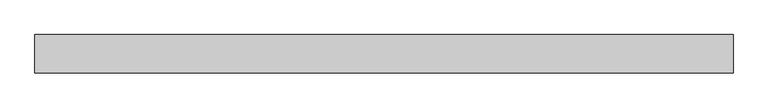
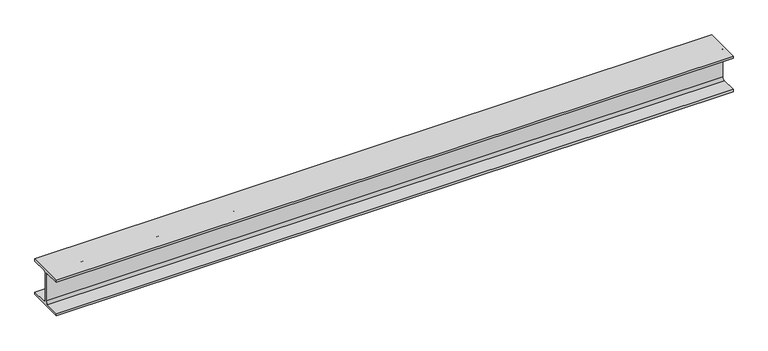
"""IFC4 building model written with IfcOpenShell, lengths in millimetres: beam geometry, 0912_Steel Framing_H-KSD3502 : H_SB_ASB_H-200x200x8x12."""

from ifc_helpers import new_model, si_unit, point, frame, frame_2d, origin, place, context, project, spatial, polyline, circle_curve, trimmed, segment, composite_curve, outline, extrude, source, transform, mapped, element, save


def beam_58b5673e(model_context):
    return source(origin(), model_context, "Body", "SweptSolid", [
        extrude(outline(composite_curve([segment(polyline([(100.0, -88.0), (100.0, -100.0), (-100.0, -100.0), (-100.0, -88.0), (-17.0, -88.0)]), True, "CONTINUOUS"), segment(trimmed(circle_curve(frame_2d((-17.0, -75.0)), 13.0), [point((-17.0, -88.0))], [point((-4.0, -75.0))], True, "CARTESIAN"), True, "CONTINUOUS"), segment(polyline([(-4.0, -75.0), (-4.0, 75.0)]), True, "CONTINUOUS"), segment(trimmed(circle_curve(frame_2d((-17.0, 75.0)), 13.0), [point((-4.0, 75.0))], [point((-17.0, 88.0))], True, "CARTESIAN"), True, "CONTINUOUS"), segment(polyline([(-17.0, 88.0), (-100.0, 88.0), (-100.0, 100.0), (100.0, 100.0), (100.0, 88.0), (17.0, 88.0)]), True, "CONTINUOUS"), segment(trimmed(circle_curve(frame_2d((17.0, 75.0)), 13.0), [point((17.0, 88.0))], [point((4.0, 75.0))], True, "CARTESIAN"), True, "CONTINUOUS"), segment(polyline([(4.0, 75.0), (4.0, -75.0)]), True, "CONTINUOUS"), segment(trimmed(circle_curve(frame_2d((17.0, -75.0)), 13.0), [point((4.0, -75.0))], [point((17.0, -88.0))], True, "CARTESIAN"), True, "CONTINUOUS"), segment(polyline([(17.0, -88.0), (100.0, -88.0)]), True, "CONTINUOUS")], self_intersect=False)), frame((-1850.8543264, 0.0, 0.0), z_axis=(1.0, 0.0, 0.0), x_axis=(0.0, 1.0, 0.0)), (0.0, 0.0, 1.0), 3630.9979746),
    ])


if __name__ == "__main__":
    model = new_model("IFC4")
    model_context = context("Model", 3, world=origin())
    ifc_project = project(units=[si_unit("LENGTHUNIT", "METRE", prefix="MILLI")], contexts=[model_context])
    site = spatial("IfcSite", under=ifc_project)
    building = spatial("IfcBuilding", under=site)
    placement = place(None, origin())
    beam_shape = beam_58b5673e(model_context)
    element("IfcBeam", 1, ObjectType="0912_Steel Framing_H-KSD3502 : H_SB_ASB_H-200x200x8x12", at=placement, inside=building, context=model_context, shape_type="MappedRepresentation", body=[
        mapped(beam_shape, transform((0.0, 0.0, 0.0), x_axis=(1.0, 0.0, 0.0), y_axis=(0.0, 1.0, 0.0), z_axis=(0.0, 0.0, 1.0))),
    ])
    save(model, "model.ifc")

# Revit data of these elements
# Type "0912_Steel Framing_H-KSD3502 : H_SB_ASB_H-200x200x8x12"
#   H_WM Code_1 = "S01AA002-00001 | Main Steel Structure Fabrication Work | Shelter/Building | Medium Steel - Standard (90KG/M>Weight≥30KG/M) | Material: (   )"
#   H_WM Code_2 = "S03AA028-00001 | Main Steel Structure Erection Work | Shelter/Building | Medium Steel (90KG/M>Weight≥30KG/M) | Material: (   )"
#   H_WM Code_3 = "S01AA010-00001 | Main Steel Structure Fabrication Work | Shelter/Building | Steel Painting/Coating | for Non-Fireproofed Steel Surface, Surface Preparation, Primer, Second & Final Coat | Material: (   )"
#   H_Q'ty Cal Type Tag = "SB-Q2"
#   Width = 20.0 cm
#   Web Thickness = 0.8 cm
#   Web Fillet = 1.3 cm
#   Warping Constant = 141000.0 cm⁶
#   W = 0
#   Torsional Moment of Inertia = 26.2485 cm⁴
#   Section Area = 63.53 cm²
#   Plastic Modulus weak axis = 244.0 cm³
#   Plastic Modulus strong axis = 525.0 cm³
#   Perimeter = 1.16 m²/m
#   Nominal Weight = 49.90 kgf/m
#   Moment of Inertia weak axis = 1600.00 cm⁴
#   Moment of Inertia strong axis = 4720.00 cm⁴
#   Height = 20.0 cm
#   Flange Thickness = 1.2 cm
#   Elastic Modulus weak axis = 160.0 cm³
#   Elastic Modulus strong axis = 472.0 cm³
#   Centroid Vertical = 10.0 cm
#   Centroid Horizontal = 10.0 cm
#   Ix = 47200000
#   Length [instance default] = 1.5240 m
#   Zx = 525000
#   b = 0.2000 m
#   h = 0.2000 m
#   r = 0.0130 m
#   s = 0.0080 m
#   t = 0.0120 m
#   A = 0.006353 m²
#   Structural Material [instance default] = Steel, 45-345
#   Assembly Code = ""
# Element 1 (IfcBeam, "0912_Steel Framing_H-KSD3502 : H_SB_ASB_H-200x200x8x12")
#   Structural Material = none
# Materials
#   "Steel, 45-345": class "Metal", colour RGB 189 187 185, transparency 0, Description = "Steel 345 MPa", Cost = 0
